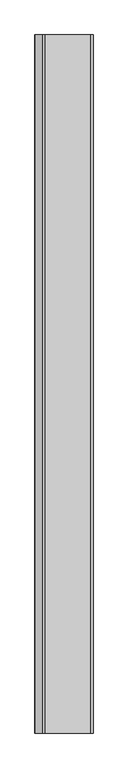
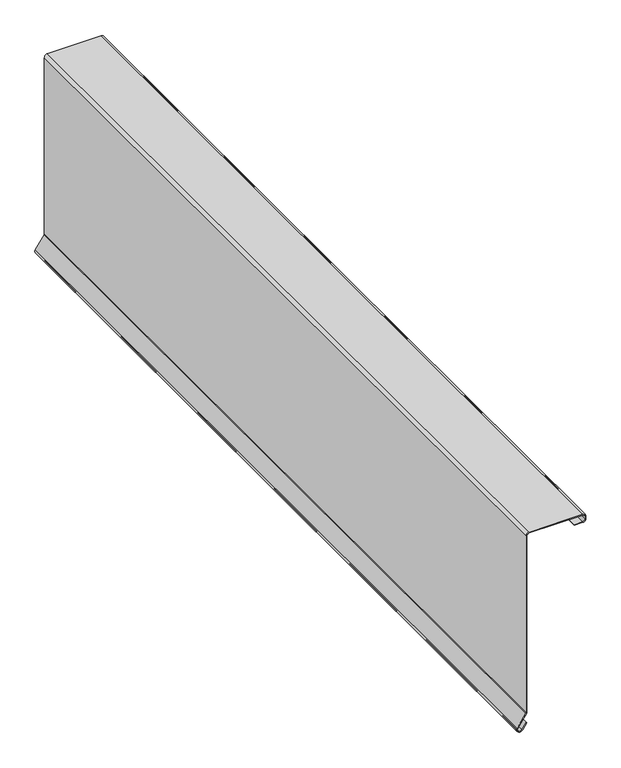
"""IFC4 building model written with IfcOpenShell, lengths in millimetres: proxy geometry, Flashing012 2990 : Flashing012 2990."""

from ifc_helpers import new_model, si_unit, point, frame, frame_2d, origin, place, context, project, spatial, polyline, circle_curve, trimmed, segment, composite_curve, outline, extrude, source, transform, mapped, element, save


def generic_models_affd795f(model_context):
    return source(origin(), model_context, "Body", "SweptSolid", [
        extrude(outline(composite_curve([segment(trimmed(circle_curve(frame_2d((42111.5532705, -2482.9530802)), 5.08), [point((42108.6312101, -2478.7976063))], [point((42107.4417652, -2485.9366895))], True, "CARTESIAN"), True, "CONTINUOUS"), segment(polyline([(42107.4417652, -2485.9366895), (42108.7344443, -2487.718041)]), True, "CONTINUOUS"), segment(trimmed(circle_curve(frame_2d((42112.8459496, -2484.7344317)), 5.08), [point((42108.7344443, -2487.718041))], [point((42115.753039, -2488.9003927))], True, "CARTESIAN"), True, "CONTINUOUS"), segment(polyline([(42115.753039, -2488.9003927), (42146.0058896, -2467.7893589)]), True, "CONTINUOUS"), segment(trimmed(circle_curve(frame_2d((42148.9129791, -2471.9553199)), 5.08), [point((42146.0058896, -2467.7893589))], [point((42148.9129791, -2466.8753199))], False, "CARTESIAN"), True, "CONTINUOUS"), segment(polyline([(42148.9129791, -2466.8753199), (42596.1419896, -2466.8753199)]), True, "CONTINUOUS"), segment(trimmed(circle_curve(frame_2d((42596.1419896, -2461.7953199)), 5.08), [point((42596.1419896, -2466.8753199))], [point((42601.2219896, -2461.7953199))], True, "CARTESIAN"), True, "CONTINUOUS"), segment(polyline([(42601.2219896, -2461.7953199), (42601.2219896, -2332.4553199)]), True, "CONTINUOUS"), segment(trimmed(circle_curve(frame_2d((42596.1419896, -2332.4553199)), 5.08), [point((42601.2219896, -2332.4553199))], [point((42596.1419896, -2327.3753199))], True, "CARTESIAN"), True, "CONTINUOUS"), segment(polyline([(42596.1419896, -2327.3753199), (42589.7355833, -2327.3753199)]), True, "CONTINUOUS"), segment(trimmed(circle_curve(frame_2d((42589.7355833, -2332.4553199)), 5.08), [point((42589.7355833, -2327.3753199))], [point((42584.6555833, -2332.4553199))], True, "CARTESIAN"), True, "CONTINUOUS"), segment(polyline([(42584.6555833, -2332.4553199), (42584.6555833, -2353.7517847), (42582.6555833, -2353.7517847), (42582.6555833, -2332.4553199)]), True, "CONTINUOUS"), segment(trimmed(circle_curve(frame_2d((42589.7355833, -2332.4553199)), 7.08), [point((42582.6555833, -2332.4553199))], [point((42589.7355833, -2325.3753199))], False, "CARTESIAN"), True, "CONTINUOUS"), segment(polyline([(42589.7355833, -2325.3753199), (42596.1419896, -2325.3753199)]), True, "CONTINUOUS"), segment(trimmed(circle_curve(frame_2d((42596.1419896, -2332.4553199)), 7.08), [point((42596.1419896, -2325.3753199))], [point((42603.2219896, -2332.4553199))], False, "CARTESIAN"), True, "CONTINUOUS"), segment(polyline([(42603.2219896, -2332.4553199), (42603.2219896, -2461.7953199)]), True, "CONTINUOUS"), segment(trimmed(circle_curve(frame_2d((42596.1419896, -2461.7953199)), 7.08), [point((42603.2219896, -2461.7953199))], [point((42596.1419896, -2468.8753199))], False, "CARTESIAN"), True, "CONTINUOUS"), segment(polyline([(42596.1419896, -2468.8753199), (42148.9129791, -2468.8753199)]), True, "CONTINUOUS"), segment(trimmed(circle_curve(frame_2d((42148.9129791, -2471.9553199)), 3.08), [point((42148.9129791, -2468.8753199))], [point((42147.150413, -2469.429501))], True, "CARTESIAN"), True, "CONTINUOUS"), segment(polyline([(42147.150413, -2469.429501), (42116.8975624, -2490.5405348)]), True, "CONTINUOUS"), segment(trimmed(circle_curve(frame_2d((42112.8459496, -2484.7344317)), 7.08), [point((42116.8975624, -2490.5405348))], [point((42107.1157415, -2488.8926904))], False, "CARTESIAN"), True, "CONTINUOUS"), segment(polyline([(42107.1157415, -2488.8926904), (42105.8230624, -2487.1113389)]), True, "CONTINUOUS"), segment(trimmed(circle_curve(frame_2d((42111.5532705, -2482.9530802)), 7.08), [point((42105.8230624, -2487.1113389))], [point((42107.4807927, -2477.161593))], False, "CARTESIAN"), True, "CONTINUOUS"), segment(polyline([(42107.4807927, -2477.161593), (42122.0676658, -2466.9043456), (42123.2180833, -2468.5403589), (42108.6312101, -2478.7976063)]), True, "CONTINUOUS")], self_intersect=False)), frame((0.0, -1052.8906574, 0.0), z_axis=(0.0, 1.0, 0.0), x_axis=(0.0, 0.0, 1.0)), (0.0, 0.0, 1.0), 2000.0),
    ])


if __name__ == "__main__":
    model = new_model("IFC4")
    model_context = context("Model", 3, world=origin())
    ifc_project = project(units=[si_unit("LENGTHUNIT", "METRE", prefix="MILLI")], contexts=[model_context])
    site = spatial("IfcSite", under=ifc_project)
    building = spatial("IfcBuilding", under=site)
    placement = place(None, origin())
    generic_models_shape = generic_models_affd795f(model_context)
    element("IfcBuildingElementProxy", 1, Name="Flashing012 2990 : Flashing012 2990", ObjectType="Flashing012 2990 : Flashing012 2990", at=placement, inside=building, context=model_context, shape_type="MappedRepresentation", body=[
        mapped(generic_models_shape, transform((0.0, 0.0, 0.0), x_axis=(1.0, 0.0, 0.0), y_axis=(0.0, 1.0, 0.0), z_axis=(0.0, 0.0, 1.0))),
    ])
    save(model, "model.ifc")

# Revit data of these elements
# Type "Flashing012 2990 : Flashing012 2990"
#   NameOverride = "Flashing012"
# Element 1 (IfcBuildingElementProxy, "Flashing012 2990 : Flashing012 2990")
#   Materials on its faces: "HIGH EAVE FLASHING"
# Materials
#   "HIGH EAVE FLASHING": class "Unassigned", colour RGB 128 128 128, transparency 0
